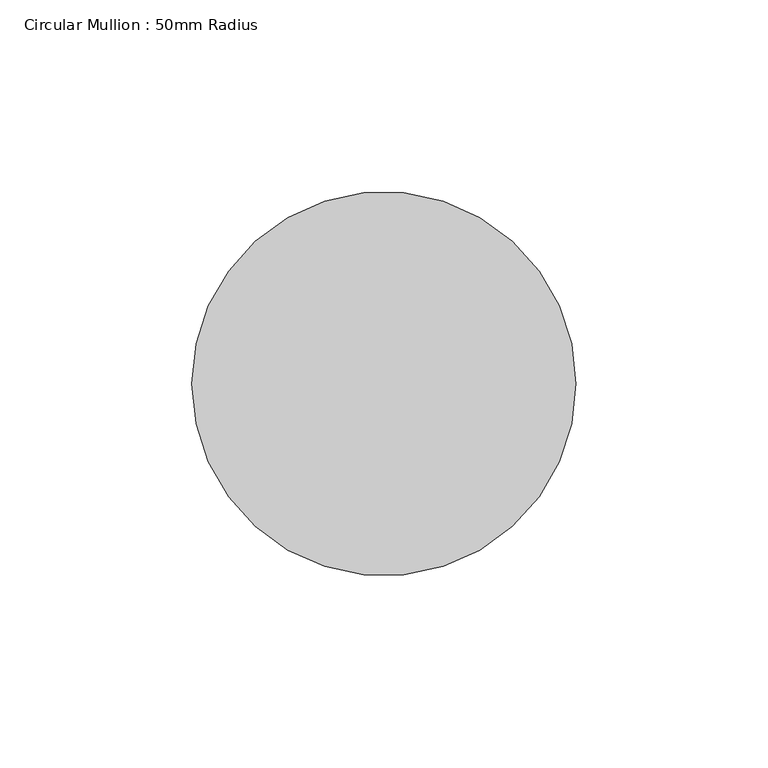
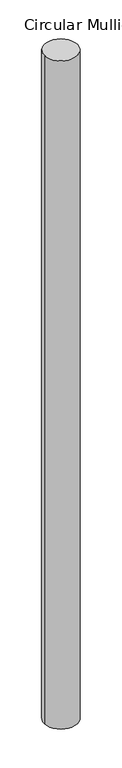
"""IFC4 building model written with IfcOpenShell, lengths in millimetres: member geometry, Circular Mullion : 50mm Radius."""

from ifc_helpers import new_model, si_unit, point, frame, frame_2d, origin, place, context, project, spatial, circle_curve, trimmed, segment, composite_curve, outline, extrude, source, transform, mapped, element, save


def circular_mullion_50mm_radius_e497fba9(model_context):
    return source(origin(), model_context, "Body", "SweptSolid", [
        extrude(outline(composite_curve([segment(trimmed(circle_curve(frame_2d((-50.0, 0.0)), 50.0), [point((0.0, 0.0))], [point((-100.0, 0.0))], False, "CARTESIAN"), True, "CONTINUOUS"), segment(trimmed(circle_curve(frame_2d((-50.0, 0.0)), 50.0), [point((-100.0, 0.0))], [point((0.0, 0.0))], False, "CARTESIAN"), True, "CONTINUOUS")], self_intersect=False)), frame((0.0, 0.0, -2124.4055645), z_axis=(0.0, 0.0, 1.0), x_axis=(1.0, 0.0, 0.0)), (0.0, 0.0, 1.0), 2124.4055645),
    ])


if __name__ == "__main__":
    model = new_model("IFC4")
    model_context = context("Model", 3, world=origin())
    ifc_project = project(units=[si_unit("LENGTHUNIT", "METRE", prefix="MILLI")], contexts=[model_context])
    site = spatial("IfcSite", under=ifc_project)
    building = spatial("IfcBuilding", under=site)
    placement = place(None, origin())
    circular_mullion_50mm_radius_shape = circular_mullion_50mm_radius_e497fba9(model_context)
    element("IfcMember", 1, ObjectType="Circular Mullion : 50mm Radius", at=placement, inside=building, context=model_context, shape_type="MappedRepresentation", body=[
        mapped(circular_mullion_50mm_radius_shape, transform((0.0, 0.0, 0.0), x_axis=(1.0, 0.0, 0.0), y_axis=(0.0, 1.0, 0.0), z_axis=(0.0, 0.0, 1.0))),
    ])
    save(model, "model.ifc")

# Revit data of these elements
# Type "Circular Mullion : 50mm Radius"
#   built-in parameter 1007350 = 0.164042 (stored number, unit not read)
# Element 1 (IfcMember, "Circular Mullion : 50mm Radius")
#   Materials on its faces: "Aluminium"
# Materials
#   "Aluminium": class "Metal", colour RGB 247 247 247, transparency 0, Description = "Aluminium 6061", Cost = 0
